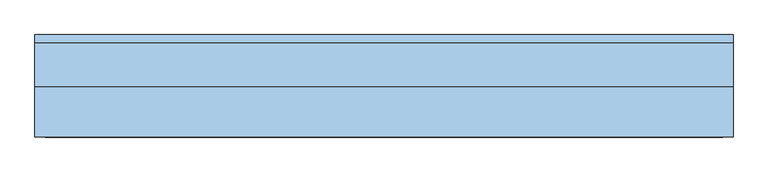
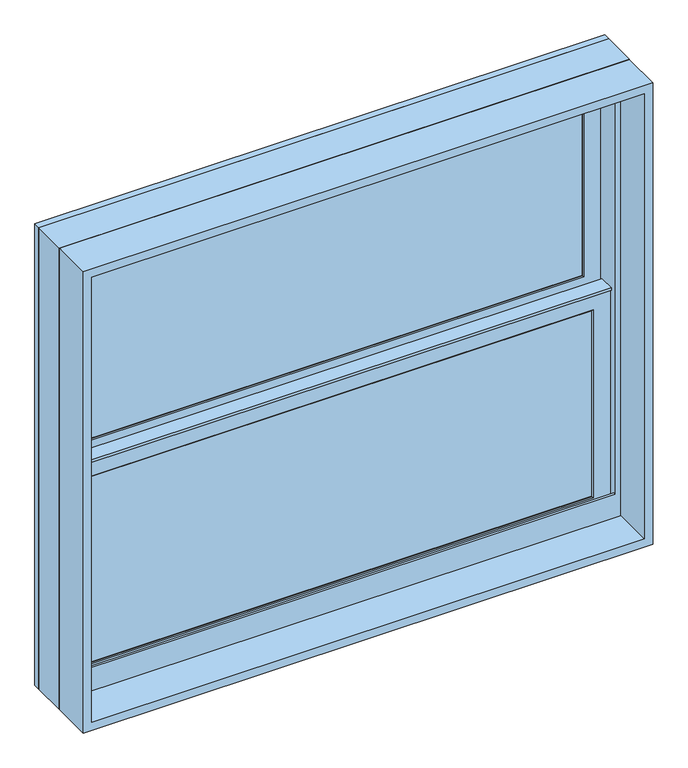
"""IFC4 building model written with IfcOpenShell, lengths in millimetres: window geometry, Window-Double_Hung-Marvin-Essential : ESDH3630."""

from ifc_helpers import new_model, si_unit, frame, origin, place, context, project, spatial, polyline, outline, extrude, faceted_brep, source, transform, mapped, element, save


def window_8936dcf3(model_context):
    return source(origin(), model_context, "Body", "SolidModel", [
        extrude(outline(polyline([(166.1583333, 20.6375), (166.1583333, 15.875), (147.1083333, 15.875), (147.1083333, 20.6375), (166.1583333, 20.6375)])), frame((0.0, 0.0, 1593.85), z_axis=(0.0, 0.0, 1.0), x_axis=(1.0, 0.0, 0.0)), (0.0, 0.0, 1.0), 374.65),
        extrude(outline(polyline([(-147.1083333, 20.6375), (-147.1083333, 15.875), (-166.1583333, 15.875), (-166.1583333, 20.6375), (-147.1083333, 20.6375)])), frame((0.0, 0.0, 1593.85), z_axis=(0.0, 0.0, 1.0), x_axis=(1.0, 0.0, 0.0)), (0.0, 0.0, 1.0), 374.65),
        extrude(outline(polyline([(469.9, 20.6375), (469.9, 15.875), (-469.9, 15.875), (-469.9, 20.6375), (469.9, 20.6375)])), frame((0.0, 0.0, 1771.65), z_axis=(0.0, 0.0, 1.0), x_axis=(1.0, 0.0, 0.0)), (0.0, 0.0, 1.0), 19.05),
        extrude(outline(polyline([(-166.1583333, 46.83125), (-166.1583333, 51.59375), (-147.1083333, 51.59375), (-147.1083333, 46.83125), (-166.1583333, 46.83125)])), frame((0.0, 0.0, 2006.6), z_axis=(0.0, 0.0, 1.0), x_axis=(1.0, 0.0, 0.0)), (0.0, 0.0, 1.0), 374.65),
        extrude(outline(polyline([(147.1083333, 46.83125), (147.1083333, 51.59375), (166.1583333, 51.59375), (166.1583333, 46.83125), (147.1083333, 46.83125)])), frame((0.0, 0.0, 2006.6), z_axis=(0.0, 0.0, 1.0), x_axis=(1.0, 0.0, 0.0)), (0.0, 0.0, 1.0), 374.65),
        extrude(outline(polyline([(-469.9, 46.83125), (-469.9, 51.59375), (469.9, 51.59375), (469.9, 46.83125), (-469.9, 46.83125)])), frame((0.0, 0.0, 2184.4), z_axis=(0.0, 0.0, 1.0), x_axis=(1.0, 0.0, 0.0)), (0.0, 0.0, 1.0), 19.05),
        extrude(outline(polyline([(166.1583333, 20.6375), (147.1083333, 20.6375), (147.1083333, 25.4), (166.1583333, 25.4), (166.1583333, 20.6375)])), frame((0.0, 0.0, 1593.85), z_axis=(0.0, 0.0, 1.0), x_axis=(1.0, 0.0, 0.0)), (0.0, 0.0, 1.0), 374.65),
        extrude(outline(polyline([(-147.1083333, 20.6375), (-166.1583333, 20.6375), (-166.1583333, 25.4), (-147.1083333, 25.4), (-147.1083333, 20.6375)])), frame((0.0, 0.0, 1593.85), z_axis=(0.0, 0.0, 1.0), x_axis=(1.0, 0.0, 0.0)), (0.0, 0.0, 1.0), 374.65),
        extrude(outline(polyline([(469.9, 20.6375), (-469.9, 20.6375), (-469.9, 25.4), (469.9, 25.4), (469.9, 20.6375)])), frame((0.0, 0.0, 1771.65), z_axis=(0.0, 0.0, 1.0), x_axis=(1.0, 0.0, 0.0)), (0.0, 0.0, 1.0), 19.05),
        extrude(outline(polyline([(-166.1583333, 56.35625), (-147.1083333, 56.35625), (-147.1083333, 51.59375), (-166.1583333, 51.59375), (-166.1583333, 56.35625)])), frame((0.0, 0.0, 2006.6), z_axis=(0.0, 0.0, 1.0), x_axis=(1.0, 0.0, 0.0)), (0.0, 0.0, 1.0), 374.65),
        extrude(outline(polyline([(147.1083333, 56.35625), (166.1583333, 56.35625), (166.1583333, 51.59375), (147.1083333, 51.59375), (147.1083333, 56.35625)])), frame((0.0, 0.0, 2006.6), z_axis=(0.0, 0.0, 1.0), x_axis=(1.0, 0.0, 0.0)), (0.0, 0.0, 1.0), 374.65),
        extrude(outline(polyline([(-469.9, 56.35625), (469.9, 56.35625), (469.9, 51.59375), (-469.9, 51.59375), (-469.9, 56.35625)])), frame((0.0, 0.0, 2184.4), z_axis=(0.0, 0.0, 1.0), x_axis=(1.0, 0.0, 0.0)), (0.0, 0.0, 1.0), 19.05),
        faceted_brep([(-496.8875, 5.6780605, 1998.5351748), (-496.8875, 5.6780605, 1993.9), (496.8875, 5.6780605, 1993.9), (496.8875, 5.6780605, 1998.5351748), (-496.8875, 34.8118605, 1998.5351748), (496.8875, 34.8118605, 1998.5351748), (496.8875, 34.8118605, 1993.9), (-496.8875, 34.8118605, 1993.9), (-496.8875, 30.1625, 1993.9), (-496.8875, 30.1625, 1566.8625), (-496.8875, 8.9241104, 1566.8625), (-496.8875, 8.9241104, 1993.9), (496.8875, 8.9241104, 1993.9), (496.8875, 30.1625, 1993.9), (496.8875, 8.9241104, 1566.8625), (496.8875, 30.1625, 1566.8625), (-481.0034752, 11.90625, 1979.6034752), (-481.0034752, 30.1625, 1979.6034752), (481.0034752, 30.1625, 1979.6034752), (481.0034752, 11.90625, 1979.6034752), (-464.34375, 10.4662439, 1962.94375), (-464.34375, 11.90625, 1962.94375), (464.34375, 11.90625, 1962.94375), (464.34375, 10.4662439, 1962.94375), (465.8858834, 8.9241104, 1964.4858834), (-465.8858834, 8.9241104, 1964.4858834), (481.0034752, 30.1625, 1582.7465248), (481.0034752, 11.90625, 1582.7465248), (464.34375, 11.90625, 1599.40625), (464.34375, 10.4662439, 1599.40625), (465.8858834, 8.9241104, 1597.8641166), (-481.0034752, 30.1625, 1582.7465248), (-481.0034752, 11.90625, 1582.7465248), (-464.34375, 11.90625, 1599.40625), (-464.34375, 10.4662439, 1599.40625), (-465.8858834, 8.9241104, 1597.8641166)], [[[0, 1, 2, 3]], [[4, 5, 6, 7]], [[1, 0, 4, 7, 8, 9, 10, 11]], [[2, 1, 11, 12]], [[7, 6, 13, 8]], [[3, 2, 12, 14, 15, 13, 6, 5]], [[0, 3, 5, 4]], [[16, 17, 18, 19]], [[20, 21, 22, 23]], [[20, 23, 24, 25]], [[19, 18, 26, 27]], [[23, 22, 28, 29]], [[24, 23, 29, 30]], [[27, 26, 31, 32]], [[29, 28, 33, 34]], [[30, 29, 34, 35]], [[15, 14, 10, 9]], [[15, 9, 8, 13], [18, 17, 31, 26]], [[17, 16, 32, 31]], [[16, 19, 27, 32], [22, 21, 33, 28]], [[21, 20, 34, 33]], [[20, 25, 35, 34]], [[10, 14, 12, 11], [25, 24, 30, 35]]]),
        extrude(outline(polyline([(38.5955581, 1979.6125), (33.5778968, 1979.6125), (33.5778968, 1981.2), (39.9405976, 1981.2), (39.9405976, 1979.6125), (61.515625, 1979.6125), (47.6307501, 1976.2975159), (38.5955581, 1976.2975159), (38.5955581, 1979.6125)])), frame((-496.8875, 0.0, 0.0), z_axis=(1.0, 0.0, 0.0), x_axis=(0.0, 1.0, 0.0)), (0.0, 0.0, 1.0), 993.775),
        faceted_brep([(527.05, 0.0, 1536.7), (527.05, 0.0, 2438.4), (-527.05, 0.0, 2438.4), (-527.05, 0.0, 1536.7), (500.85625, 0.0, 1597.81875), (-500.85625, 0.0, 1597.81875), (-500.85625, 0.0, 2412.20625), (500.85625, 0.0, 2412.20625), (500.85625, 3.96875, 1536.7), (-500.85625, 3.96875, 1536.7), (-500.85625, 3.96875, 1597.81875), (500.85625, 3.96875, 1597.81875), (-527.05, 65.6828125, 1536.7), (-500.85625, 65.6828125, 1536.7), (500.85625, 65.6828125, 1536.7), (527.05, 65.6828125, 1536.7), (-527.05, 65.6828125, 2438.4), (527.05, 65.6828125, 2438.4), (500.85625, 65.6828125, 2412.20625), (-500.85625, 65.6828125, 2412.20625)], [[[0, 1, 2, 3], [4, 5, 6, 7]], [[8, 9, 10, 11]], [[5, 4, 11, 10]], [[0, 3, 12, 13, 9, 8, 14, 15]], [[13, 12, 16, 17, 15, 14, 18, 19]], [[13, 19, 6, 5, 10, 9]], [[7, 6, 19, 18]], [[18, 14, 8, 11, 4, 7]], [[1, 0, 15, 17]], [[2, 1, 17, 16]], [[3, 2, 16, 12]]]),
        faceted_brep([(500.85625, 30.1625, 1987.55), (499.26875, 30.1625, 1987.55), (499.26875, 30.1625, 1561.0544613), (500.85625, 30.1625, 1561.0544613), (-499.26875, 30.1625, 1987.55), (-500.85625, 30.1625, 1987.55), (-500.85625, 30.1625, 1561.0544613), (-499.26875, 30.1625, 1561.0544613), (499.26875, 63.5, 1987.55), (500.85625, 63.5, 1987.55), (500.85625, 63.5, 1554.5743077), (499.26875, 63.5, 1554.5743077), (-500.85625, 63.5, 1987.55), (-499.26875, 63.5, 1987.55), (-499.26875, 63.5, 1554.5743077), (-500.85625, 63.5, 1554.5743077), (512.1108932, 3.96875, 1566.1460105), (512.1108932, 3.96875, 1536.7), (512.1108932, 65.6828125, 1536.7), (512.1108932, 65.6828125, 1554.150012), (-512.1108932, 3.96875, 1536.7), (-512.1108932, 3.96875, 1566.1460105), (-512.1108932, 65.6828125, 1554.150012), (-512.1108932, 65.6828125, 1536.7), (512.1108932, 78.58125, 1551.6428097), (-512.1108932, 78.58125, 1551.6428097), (-510.0971252, 68.2348864, 1553.6539391), (-492.13135, 68.2348864, 1553.6539391), (-492.13135, 65.6828125, 1554.150012), (492.13135, 65.6828125, 1554.150012), (492.13135, 68.2348864, 1553.6539391), (510.0971252, 68.2348864, 1553.6539391), (-527.05, 65.6828125, 1536.7), (-527.05, 78.5948249, 1536.7), (527.05, 78.5948249, 1536.7), (527.05, 65.6828125, 1536.7), (-527.05, 78.58125, 2438.4), (527.05, 78.58125, 2438.4), (512.1108932, 78.58125, 2423.4608932), (-512.1108932, 78.58125, 2423.4608932), (-527.05, 65.6828125, 2438.4), (-510.0971252, 68.2348864, 2421.4471252), (510.0971252, 68.2348864, 2421.4471252), (492.13135, 68.2348864, 2403.48135), (-492.13135, 68.2348864, 2403.48135), (-492.13135, 65.6828125, 2403.48135), (492.13135, 65.6828125, 2403.48135), (527.05, 65.6828125, 2438.4)], [[[0, 1, 2, 3]], [[4, 5, 6, 7]], [[8, 9, 10, 11]], [[12, 13, 14, 15]], [[1, 8, 11, 2]], [[9, 0, 3, 10]], [[1, 0, 9, 8]], [[5, 4, 13, 12]], [[5, 12, 15, 6]], [[13, 4, 7, 14]], [[16, 17, 18, 19]], [[20, 21, 22, 23]], [[24, 25, 26, 27, 28, 22, 21, 16, 19, 29, 30, 31], [3, 2, 11, 10], [7, 6, 15, 14]], [[17, 16, 21, 20]], [[17, 20, 23, 32, 33, 34, 35, 18]], [[34, 33, 36, 37], [25, 24, 38, 39]], [[33, 32, 40, 36]], [[39, 41, 26, 25]], [[41, 42, 31, 30, 43, 44, 27, 26]], [[44, 45, 28, 27]], [[40, 32, 23, 22, 28, 45, 46, 29, 19, 18, 35, 47]], [[36, 40, 47, 37]], [[39, 38, 42, 41]], [[44, 43, 46, 45]], [[34, 37, 47, 35]], [[42, 38, 24, 31]], [[46, 43, 30, 29]]]),
        extrude(outline(polyline([(477.04375, 11.90625), (-477.04375, 11.90625), (-477.04375, 15.08125), (477.04375, 15.08125), (477.04375, 11.90625)])), frame((0.0, 0.0, 1586.70625), z_axis=(0.0, 0.0, 1.0), x_axis=(1.0, 0.0, 0.0)), (0.0, 0.0, 1.0), 388.9375),
        extrude(outline(polyline([(477.04375, 42.8625), (-477.04375, 42.8625), (-477.04375, 46.0375), (477.04375, 46.0375), (477.04375, 42.8625)])), frame((0.0, 0.0, 1999.45625), z_axis=(0.0, 0.0, 1.0), x_axis=(1.0, 0.0, 0.0)), (0.0, 0.0, 1.0), 388.9375),
        faceted_brep([(-464.34375, 31.194477, 1962.94375), (-465.8858834, 32.7366104, 1964.4858834), (465.8858834, 32.7366104, 1964.4858834), (464.34375, 31.194477, 1962.94375), (-464.34375, 30.1625, 1962.94375), (464.34375, 30.1625, 1962.94375), (-496.8875, 32.7366104, 1995.4875), (-496.8875, 30.1625, 1995.4875), (496.8875, 30.1625, 1995.4875), (496.8875, 32.7366104, 1995.4875), (465.8858834, 32.7366104, 1597.8641166), (464.34375, 31.194477, 1599.40625), (464.34375, 30.1625, 1599.40625), (496.8875, 30.1625, 1566.8625), (496.8875, 32.7366104, 1566.8625), (-465.8858834, 32.7366104, 1597.8641166), (-464.34375, 31.194477, 1599.40625), (-464.34375, 30.1625, 1599.40625), (-496.8875, 30.1625, 1566.8625), (-496.8875, 32.7366104, 1566.8625)], [[[0, 1, 2, 3]], [[4, 0, 3, 5]], [[6, 7, 8, 9]], [[3, 2, 10, 11]], [[5, 3, 11, 12]], [[9, 8, 13, 14]], [[11, 10, 15, 16]], [[12, 11, 16, 17]], [[14, 13, 18, 19]], [[9, 14, 19, 6], [1, 15, 10, 2]], [[16, 15, 1, 0]], [[17, 16, 0, 4]], [[7, 18, 13, 8], [5, 12, 17, 4]], [[19, 18, 7, 6]]]),
        faceted_brep([(-481.0034752, 42.8625, 2392.3534752), (-481.0034752, 61.11875, 2392.3534752), (481.0034752, 61.11875, 2392.3534752), (481.0034752, 42.8625, 2392.3534752), (-464.34375, 41.4224939, 2375.69375), (-464.34375, 42.8625, 2375.69375), (464.34375, 42.8625, 2375.69375), (464.34375, 41.4224939, 2375.69375), (-465.8858834, 39.8803604, 2377.2358834), (465.8858834, 39.8803604, 2377.2358834), (-496.8875, 61.11875, 2408.2375), (-496.8875, 39.8803604, 2408.2375), (496.8875, 39.8803604, 2408.2375), (496.8875, 61.11875, 2408.2375), (481.0034752, 61.11875, 1995.4965248), (481.0034752, 42.8625, 1995.4965248), (464.34375, 42.8625, 2012.15625), (464.34375, 41.4224939, 2012.15625), (465.8858834, 39.8803604, 2010.6141166), (496.8875, 39.8803604, 1979.6125), (496.8875, 61.11875, 1979.6125), (-481.0034752, 61.11875, 1995.4965248), (-481.0034752, 42.8625, 1995.4965248), (-464.34375, 42.8625, 2012.15625), (-464.34375, 41.4224939, 2012.15625), (-465.8858834, 39.8803604, 2010.6141166), (-496.8875, 39.8803604, 1979.6125), (-496.8875, 61.11875, 1979.6125)], [[[0, 1, 2, 3]], [[4, 5, 6, 7]], [[8, 4, 7, 9]], [[10, 11, 12, 13]], [[3, 2, 14, 15]], [[7, 6, 16, 17]], [[9, 7, 17, 18]], [[13, 12, 19, 20]], [[15, 14, 21, 22]], [[17, 16, 23, 24]], [[18, 17, 24, 25]], [[20, 19, 26, 27]], [[13, 20, 27, 10], [1, 21, 14, 2]], [[22, 21, 1, 0]], [[3, 15, 22, 0], [5, 23, 16, 6]], [[24, 23, 5, 4]], [[25, 24, 4, 8]], [[11, 26, 19, 12], [9, 18, 25, 8]], [[27, 26, 11, 10]]]),
        faceted_brep([(-496.8875, 61.11875, 1979.6125), (-496.8875, 63.6928604, 1979.6125), (496.8875, 63.6928604, 1979.6125), (496.8875, 61.11875, 1979.6125), (-464.34375, 62.150727, 2012.15625), (-464.34375, 61.11875, 2012.15625), (464.34375, 61.11875, 2012.15625), (464.34375, 62.150727, 2012.15625), (-465.8858834, 63.6928604, 2010.6141166), (465.8858834, 63.6928604, 2010.6141166), (496.8875, 63.6928604, 2408.2375), (496.8875, 61.11875, 2408.2375), (464.34375, 61.11875, 2375.69375), (464.34375, 62.150727, 2375.69375), (465.8858834, 63.6928604, 2377.2358834), (-496.8875, 63.6928604, 2408.2375), (-496.8875, 61.11875, 2408.2375), (-464.34375, 61.11875, 2375.69375), (-464.34375, 62.150727, 2375.69375), (-465.8858834, 63.6928604, 2377.2358834)], [[[0, 1, 2, 3]], [[4, 5, 6, 7]], [[8, 4, 7, 9]], [[3, 2, 10, 11]], [[7, 6, 12, 13]], [[9, 7, 13, 14]], [[11, 10, 15, 16]], [[13, 12, 17, 18]], [[14, 13, 18, 19]], [[16, 15, 1, 0]], [[3, 11, 16, 0], [5, 17, 12, 6]], [[18, 17, 5, 4]], [[19, 18, 4, 8]], [[1, 15, 10, 2], [9, 14, 19, 8]]]),
        extrude(outline(polyline([(477.04375, 26.19375), (-477.04375, 26.19375), (-477.04375, 30.1625), (477.04375, 30.1625), (477.04375, 26.19375)])), frame((0.0, 0.0, 1586.70625), z_axis=(0.0, 0.0, 1.0), x_axis=(1.0, 0.0, 0.0)), (0.0, 0.0, 1.0), 388.9375),
        extrude(outline(polyline([(477.04375, 57.15), (-477.04375, 57.15), (-477.04375, 61.11875), (477.04375, 61.11875), (477.04375, 57.15)])), frame((0.0, 0.0, 1999.45625), z_axis=(0.0, 0.0, 1.0), x_axis=(1.0, 0.0, 0.0)), (0.0, 0.0, 1.0), 388.9375),
        extrude(outline(polyline([(2438.4, 527.05), (2438.4, -527.05), (1536.7, -527.05), (1536.7, 527.05), (2438.4, 527.05)]), holes=[polyline([(2422.525, 511.175), (1552.575, 511.175), (1552.575, -511.175), (2422.525, -511.175), (2422.525, 511.175)])]), frame((0.0, -76.2, 0.0), z_axis=(0.0, 1.0, 0.0), x_axis=(0.0, 0.0, 1.0)), (0.0, 0.0, 1.0), 75.40625),
    ])


if __name__ == "__main__":
    model = new_model("IFC4")
    model_context = context("Model", 3, world=origin())
    ifc_project = project(units=[si_unit("LENGTHUNIT", "METRE", prefix="MILLI")], contexts=[model_context])
    site = spatial("IfcSite", under=ifc_project)
    building = spatial("IfcBuilding", under=site)
    placement = place(None, origin())
    window_shape = window_8936dcf3(model_context)
    element("IfcWindow", 1, ObjectType="Window-Double_Hung-Marvin-Essential : ESDH3630", at=placement, inside=building, context=model_context, shape_type="MappedRepresentation", body=[
        mapped(window_shape, transform((0.0, 0.0, 0.0), x_axis=(1.0, 0.0, 0.0), y_axis=(0.0, 1.0, 0.0), z_axis=(0.0, 0.0, 1.0))),
    ])
    save(model, "model.ifc")

# Revit data of these elements
# Type "Window-Double_Hung-Marvin-Essential : ESDH3630"
#   Type Mark = "38"
#   Window Type = "Essential Double Hung"
#   Product data url = "https://bimobject.com/marvin-windows-and-doors/product/marvin-dhwau"
#   Product Guid = "c4a96547-874c-4385-91dc-a058adc19d98"
#   Frame = "All Ultrex"
#   Egress Window = "No"
#   URL = "www.marvin.com"
#   Model = "ESDH3630"
#   Manufacturer = "Marvin Windows and Doors"
#   Label Egress = ""
#   Glass Type = "IG Low E II with Argon"
#   Design Pressure = "DP50"
#   Description = "4236 DBHG"
#   Analytic Construction = "<None>"
#   Prairie Corner Width = 0' - 4"
#   Prairie Corner Height = 0' - 4"
#   Egress Width = 3' - 2 9/16"
#   Egress Height = 1' - 1 27/128"
#   Rough Width = 3' - 6"
#   Rough Height = 3' - 0"
#   Nominal Width = 3' - 6"
#   Nominal Height = 3' - 0"
#   Inset to Installation Flange [instance default] = 0' - 1"
#   Height = 2' - 11 1/2"
#   Egress Area = 3.53782 SF
#   Default Head Height = 8' - 0"
#   Width = 3' - 5 1/2"
#   Daylight Area = 7.26807 SF
#   DLO Width = 3' - 0 9/16"
#   DLO Height = 1' - 2 5/16"
#   Muntins Top Sash = yes
#   Lites Wide Top Sash = 3
#   Lites Wide Bottom Sash = 3
#   Lites High Top Sash = 2
#   Lites High Bottom Sash = 2
#   Lite Cut Prairie 9 = no
#   Lite Cut HV Grid = yes
#   Muntins Bottom Sash = yes
#   Label Visibility = no
#   Jamb Extension Visibility = yes
#   Edition number = 1
#   Interior Material = Ultrex-Marvin-Stonewhite
#   Glazing Material = Glass-Marvin-IG Low E II with Argon
#   Cladding Material = Ultrex-Marvin-Pebblegray
#   Wall Closure = (empty or 0)
#   Assembly Code = ""
# Element 1 (IfcWindow, "Window-Double_Hung-Marvin-Essential : ESDH3630")
#   Materials on its faces: "Ultrex-Marvin-Pebblegray", "Ultrex-Marvin-Stonewhite", "Glass-Marvin-IG Low E II with Argon"
# Materials
#   "Ultrex-Marvin-Stonewhite": class "Paint", colour RGB 250 251 245, transparency 0
#   "Glass-Marvin-IG Low E II with Argon": class "Glass", colour RGB 0 128 192, transparency 0.85
#   "Ultrex-Marvin-Pebblegray": class "Paint", colour RGB 189 185 173, transparency 0
